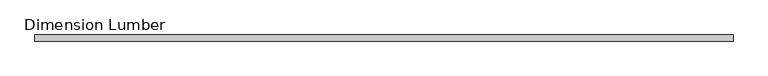
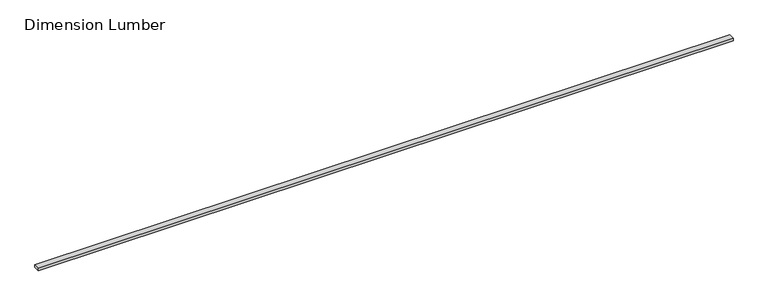
"""IFC4 building model written with IfcOpenShell, lengths in millimetres: beam geometry, Dimension Lumber : Top Supporting Lumbers."""

import ifcopenshell
import ifcopenshell.guid

model = None  # the IFC model being written
_history = None  # IfcOwnerHistory: only IFC2X3 demands one
_inside = {}  # id of a spatial element -> (the spatial element, [elements in it])
_under = {}  # id of a project, library or spatial element -> (it, [spatial elements below it])
_declared = {}  # id of a project -> (the project, [libraries it declares])
_typed = {}  # id of a type object -> (the type object, [elements of that type])
_made_of = {}  # id of a material, layer set ... -> (it, [elements and type objects made of it])


def new_model(schema):
    """Start an empty IFC model of exactly this schema.

    Asked for "IFC4X3", IfcOpenShell would pick the latest addendum, in which some entities
    have other attributes; the version numbers below select the first issue.
    IFC2X3 requires an IfcOwnerHistory on every rooted entity: one is made here for all.
    """
    global model, _history
    if schema == "IFC4X3":
        model = ifcopenshell.file(schema_version=(4, 3, 0, 0))
    else:
        model = ifcopenshell.file(schema=schema)
    _inside.clear()
    _under.clear()
    _declared.clear()
    _typed.clear()
    _made_of.clear()
    _history = None
    if model.schema == "IFC2X3":
        org = make("IfcOrganization", Name="unknown")
        user = make(
            "IfcPersonAndOrganization",
            ThePerson=make("IfcPerson", FamilyName="unknown"),
            TheOrganization=org,
        )
        app = make(
            "IfcApplication",
            ApplicationDeveloper=org,
            Version="unknown",
            ApplicationFullName="unknown",
            ApplicationIdentifier="unknown",
        )
        _history = make(
            "IfcOwnerHistory",
            OwningUser=user,
            OwningApplication=app,
            ChangeAction="ADDED",
            CreationDate=0,
        )
    return model


def make(cls, **values):
    """One entity of the class cls with the attributes given. An attribute that is None is left unset."""
    return model.create_entity(
        cls, **{name: value for name, value in values.items() if value is not None}
    )


def rooted(cls, **values):
    """An entity with a GlobalId (a new one), such as an element, a storey or a relation."""
    return make(cls, GlobalId=ifcopenshell.guid.new(), OwnerHistory=_history, **values)


def si_unit(unit_type, name, prefix=None):
    """IfcSIUnit, for example si_unit("LENGTHUNIT", "METRE", prefix="MILLI")."""
    return make("IfcSIUnit", UnitType=unit_type, Prefix=prefix, Name=name)


def assignment(units):
    """IfcUnitAssignment: the units of a project."""
    return None if units is None else make("IfcUnitAssignment", Units=units)


def point(xyz):
    """IfcCartesianPoint."""
    return None if xyz is None else make("IfcCartesianPoint", Coordinates=xyz)


def direction(xyz):
    """IfcDirection."""
    return None if xyz is None else make("IfcDirection", DirectionRatios=xyz)


def frame(location, z_axis=None, x_axis=None):
    """IfcAxis2Placement3D, a coordinate frame: its origin and axes. An axis left out is left unset."""
    return make(
        "IfcAxis2Placement3D",
        Location=point(location),
        Axis=direction(z_axis),
        RefDirection=direction(x_axis),
    )


def origin():
    """The frame at (0, 0, 0) with its axes left unset."""
    return frame((0.0, 0.0, 0.0))


def place(relative_to, where):
    """IfcLocalPlacement: puts the frame where relative to a parent placement (None: the world)."""
    return make(
        "IfcLocalPlacement", PlacementRelTo=relative_to, RelativePlacement=where
    )


def context(
    kind, dimensions, precision=None, world=None, true_north=None, identifier=None
):
    """IfcGeometricRepresentationContext, for example the 3D "Model" context."""
    return make(
        "IfcGeometricRepresentationContext",
        ContextIdentifier=identifier,
        ContextType=kind,
        CoordinateSpaceDimension=dimensions,
        Precision=precision,
        WorldCoordinateSystem=world,
        TrueNorth=true_north,
    )


def project(units=None, contexts=None):
    """IfcProject with its units and contexts."""
    return rooted(
        "IfcProject",
        Name="project",
        RepresentationContexts=contexts,
        UnitsInContext=assignment(units),
    )


def spatial(cls, under=None, at=None, **own):
    """A site, building, storey or space (cls), placed at a placement, below another one or the project."""
    s = rooted(cls, ObjectPlacement=at, **own)
    if under is not None:
        _under.setdefault(under.id(), (under, []))[1].append(s)
    return s


def polyline(points):
    """IfcPolyline through the points."""
    return make("IfcPolyline", Points=[point(p) for p in points])


def outline(outer, holes=None, kind="AREA"):
    """IfcArbitraryClosedProfileDef: a profile drawn as a closed curve; with holes, ...WithVoids."""
    if holes is None:
        return make("IfcArbitraryClosedProfileDef", ProfileType=kind, OuterCurve=outer)
    return make(
        "IfcArbitraryProfileDefWithVoids",
        ProfileType=kind,
        OuterCurve=outer,
        InnerCurves=holes,
    )


def extrude(swept, where, along, depth):
    """IfcExtrudedAreaSolid: the profile swept, set in the frame where, extruded along a direction by depth."""
    return make(
        "IfcExtrudedAreaSolid",
        SweptArea=swept,
        Position=where,
        ExtrudedDirection=direction(along),
        Depth=depth,
    )


def shape(context_of_items, identifier, shape_type, items):
    """IfcShapeRepresentation: the items that make up one representation, for example the "Body"."""
    return make(
        "IfcShapeRepresentation",
        ContextOfItems=context_of_items,
        RepresentationIdentifier=identifier,
        RepresentationType=shape_type,
        Items=items,
    )


def source(mapping_origin, context_of_items, identifier, shape_type, items):
    """IfcRepresentationMap: a shape defined once, which mapped items show again and again."""
    return make(
        "IfcRepresentationMap",
        MappingOrigin=mapping_origin,
        MappedRepresentation=shape(context_of_items, identifier, shape_type, items),
    )


def transform(
    local_origin,
    x_axis=None,
    y_axis=None,
    z_axis=None,
    scale=None,
    scale2=None,
    scale3=None,
    uniform=True,
):
    """IfcCartesianTransformationOperator3D, or its non-uniform kind. x_axis, y_axis, z_axis: its Axis1, 2, 3."""
    if uniform:
        return make(
            "IfcCartesianTransformationOperator3D",
            Axis1=direction(x_axis),
            Axis2=direction(y_axis),
            LocalOrigin=point(local_origin),
            Scale=scale,
            Axis3=direction(z_axis),
        )
    return make(
        "IfcCartesianTransformationOperator3DnonUniform",
        Axis1=direction(x_axis),
        Axis2=direction(y_axis),
        LocalOrigin=point(local_origin),
        Scale=scale,
        Axis3=direction(z_axis),
        Scale2=scale2,
        Scale3=scale3,
    )


def mapped(mapping_source, mapping_target):
    """IfcMappedItem: shows the shape of a source again, moved by a transform."""
    return make(
        "IfcMappedItem", MappingSource=mapping_source, MappingTarget=mapping_target
    )


def made_of(thing, what):
    """Note that an element or type object is made of a material, layer set ...; save() writes the relation."""
    if what is not None:
        _made_of.setdefault(what.id(), (what, []))[1].append(thing)
    return thing


def element(
    cls,
    number,
    at=None,
    inside=None,
    cuts=None,
    type_object=None,
    material=None,
    context=None,
    identifier="Body",
    shape_type=None,
    held_by="IfcProductDefinitionShape",
    body=None,
    shapes=None,
    **own,
):
    """One element of the class cls, such as IfcWall. Its Tag is "e" and its number.

    at: its placement. inside: the storey or other place that contains it. cuts: it is an
    opening in that element (IfcRelVoidsElement). A single representation is given by context,
    identifier, shape_type and body (its items); several are given by shapes. held_by: the class
    of the entity that holds the representations. save() writes the other relations.
    """
    e = rooted(cls, Tag="e%d" % number, ObjectPlacement=at, **own)
    if body is not None:
        shapes = [shape(context, identifier, shape_type, body)]
    if shapes is not None:
        e.Representation = make(held_by, Representations=shapes)
    if inside is not None:
        _inside.setdefault(inside.id(), (inside, []))[1].append(e)
    if cuts is not None:
        rooted(
            "IfcRelVoidsElement", RelatingBuildingElement=cuts, RelatedOpeningElement=e
        )
    if type_object is not None:
        _typed.setdefault(type_object.id(), (type_object, []))[1].append(e)
    return made_of(e, material)


def aggregate(whole, parts):
    """IfcRelAggregates: a whole, such as a stair, and the parts it consists of."""
    return rooted("IfcRelAggregates", RelatingObject=whole, RelatedObjects=parts)


def save(model, path):
    """Write the relations noted so far, then the file.

    IfcRelAggregates (storeys below a building ...), IfcRelContainedInSpatialStructure (elements
    in a storey), IfcRelDefinesByType, IfcRelAssociatesMaterial and IfcRelDeclares: one each for
    every whole, place, type object, material and project.
    """
    for whole, parts in _under.values():
        aggregate(whole, parts)
    for where, things in _inside.values():
        rooted(
            "IfcRelContainedInSpatialStructure",
            RelatedElements=things,
            RelatingStructure=where,
        )
    for kind, things in _typed.values():
        rooted("IfcRelDefinesByType", RelatedObjects=things, RelatingType=kind)
    for what, things in _made_of.values():
        rooted("IfcRelAssociatesMaterial", RelatedObjects=things, RelatingMaterial=what)
    for by, libraries in _declared.values():
        rooted("IfcRelDeclares", RelatingContext=by, RelatedDefinitions=libraries)
    model.write(path)


def dimension_lumber_4f6bd669(model_context):
    return source(origin(), model_context, "Body", "SweptSolid", [
        extrude(outline(polyline([(5017.29375, 44.45), (5017.29375, -44.45), (-5144.29375, -44.45), (-5144.29375, 44.45), (5017.29375, 44.45)])), frame((0.0, 0.0, -19.05), z_axis=(0.0, 0.0, 1.0), x_axis=(1.0, 0.0, 0.0)), (0.0, 0.0, 1.0), 38.1),
    ])


if __name__ == "__main__":
    model = new_model("IFC4")
    model_context = context("Model", 3, world=origin())
    ifc_project = project(units=[si_unit("LENGTHUNIT", "METRE", prefix="MILLI")], contexts=[model_context])
    site = spatial("IfcSite", under=ifc_project)
    building = spatial("IfcBuilding", under=site)
    placement = place(None, origin())
    dimension_lumber_shape = dimension_lumber_4f6bd669(model_context)
    element("IfcBeam", 1, ObjectType="Dimension Lumber : Top Supporting Lumbers", at=placement, inside=building, context=model_context, shape_type="MappedRepresentation", body=[
        mapped(dimension_lumber_shape, transform((0.0, 0.0, 0.0), x_axis=(1.0, 0.0, 0.0), y_axis=(0.0, 1.0, 0.0), z_axis=(0.0, 0.0, 1.0))),
    ])
    save(model, "model.ifc")

# Revit data of these elements
# Type "Dimension Lumber : Top Supporting Lumbers"
#   Assembly Code = "B10"
#   A = 0.0364583 SF
#   Length [instance default] = 5' - 0"
#   b = 0' - 3 1/2"
#   d = 0' - 1 1/2"
#   Structural Material [instance default] = Softwood, Lumber
# Element 1 (IfcBeam, "Dimension Lumber : Top Supporting Lumbers")
#   Structural Material = Douglas Fir #2
#   Materials on its faces: "Douglas Fir #2"
# Materials
#   "Softwood, Lumber": class "Wood", colour RGB 223 192 134, transparency 0, Description = "Pinus Echinata", Cost = 0
#   "Douglas Fir #2": class "Wood", colour RGB 223 192 134, transparency 0, Description = "Pinus Echinata", Cost = 0
